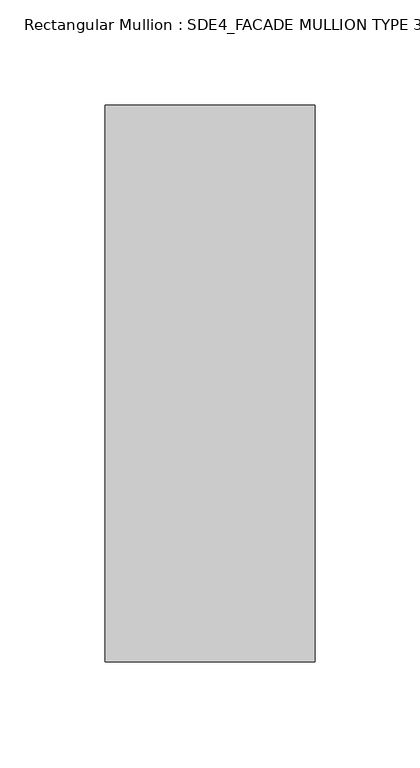
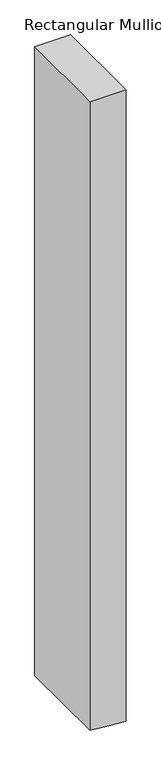
"""IFC4 building model written with IfcOpenShell, lengths in millimetres: member geometry, Rectangular Mullion : SDE4_FACADE MULLION TYPE 3."""

from ifc_helpers import new_model, si_unit, frame, origin, place, context, project, spatial, polyline, outline, extrude, source, transform, mapped, element, save


def rectangular_mullion_sde4_facade_mullion_type_3_89046874(model_context):
    return source(origin(), model_context, "Body", "SweptSolid", [
        extrude(outline(polyline([(0.0, 50.0), (0.0, -50.0), (-1843.9366009, -50.0), (-1848.00268, 3.056508), (-1851.6002773, 50.0), (0.0, 50.0)])), frame((0.0, -132.5, 0.0), z_axis=(0.0, 1.0, 0.0), x_axis=(0.0, 0.0, 1.0)), (0.0, 0.0, 1.0), 265.0),
    ])


if __name__ == "__main__":
    model = new_model("IFC4")
    model_context = context("Model", 3, world=origin())
    ifc_project = project(units=[si_unit("LENGTHUNIT", "METRE", prefix="MILLI")], contexts=[model_context])
    site = spatial("IfcSite", under=ifc_project)
    building = spatial("IfcBuilding", under=site)
    placement = place(None, origin())
    rectangular_mullion_sde4_facade_mullion_type_3_shape = rectangular_mullion_sde4_facade_mullion_type_3_89046874(model_context)
    element("IfcMember", 1, ObjectType="Rectangular Mullion : SDE4_FACADE MULLION TYPE 3", at=placement, inside=building, context=model_context, shape_type="MappedRepresentation", body=[
        mapped(rectangular_mullion_sde4_facade_mullion_type_3_shape, transform((0.0, 0.0, 0.0), x_axis=(1.0, 0.0, 0.0), y_axis=(0.0, 1.0, 0.0), z_axis=(0.0, 0.0, 1.0))),
    ])
    save(model, "model.ifc")

# Revit data of these elements
# Type "Rectangular Mullion : SDE4_FACADE MULLION TYPE 3"
#   built-in parameter 1007322 = 0.869423 (stored number, unit not read)
#   built-in parameter 1007321 = 0.164042 (stored number, unit not read)
#   built-in parameter 1007320 = 0.164042 (stored number, unit not read)
